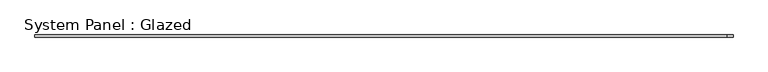
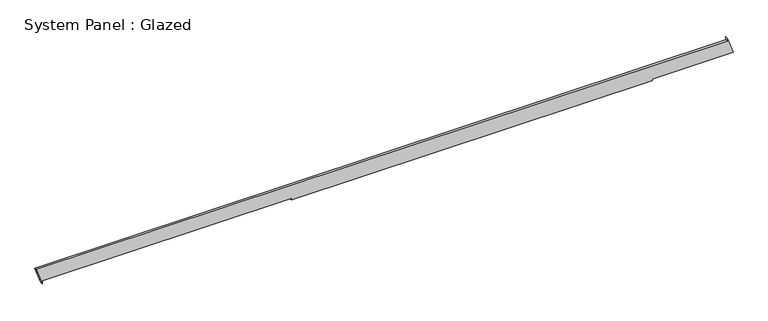
"""IFC4 building model written with IfcOpenShell, lengths in millimetres: plate geometry, System Panel : Glazed."""

from ifc_helpers import new_model, si_unit, frame, origin, place, context, project, spatial, polyline, outline, extrude, source, transform, mapped, element, save


def system_panel_glazed_82b7ec84(model_context):
    return source(origin(), model_context, "Body", "SweptSolid", [
        extrude(outline(polyline([(0.0, -3959.3382367), (35.3553391, -3959.3382367), (35.3553391, -1080.0643239), (19.2141513, -1079.589913), (19.2159629, 3093.0829852), (35.3553391, 3094.3752998), (35.3553391, 4027.9814555), (234.8084044, 3959.4408873), (199.4530653, 3959.4410749), (199.4106846, -4027.9814555), (0.0, -3959.3382367)])), frame((0.0, -49.5, 0.0), z_axis=(0.0, 1.0, 0.0), x_axis=(0.0, 0.0, 1.0)), (0.0, 0.0, 1.0), 25.0),
    ])


if __name__ == "__main__":
    model = new_model("IFC4")
    model_context = context("Model", 3, world=origin())
    ifc_project = project(units=[si_unit("LENGTHUNIT", "METRE", prefix="MILLI")], contexts=[model_context])
    site = spatial("IfcSite", under=ifc_project)
    building = spatial("IfcBuilding", under=site)
    placement = place(None, origin())
    system_panel_glazed_shape = system_panel_glazed_82b7ec84(model_context)
    element("IfcPlate", 1, ObjectType="System Panel : Glazed", at=placement, inside=building, context=model_context, shape_type="MappedRepresentation", body=[
        mapped(system_panel_glazed_shape, transform((0.0, 0.0, 0.0), x_axis=(1.0, 0.0, 0.0), y_axis=(0.0, 1.0, 0.0), z_axis=(0.0, 0.0, 1.0))),
    ])
    save(model, "model.ifc")

# Revit data of these elements
# Element 1 (IfcPlate, "System Panel : Glazed")
#   Materials on its faces: "Glass"
# Materials
#   "Glass": class "Glass", colour RGB 218 227 224, transparency 0.85, Description = "Soda Lime Glass", Cost = 0
